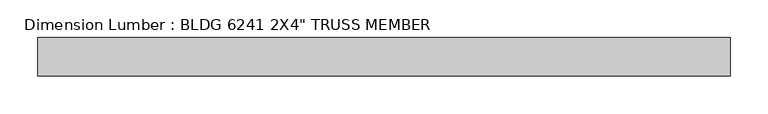
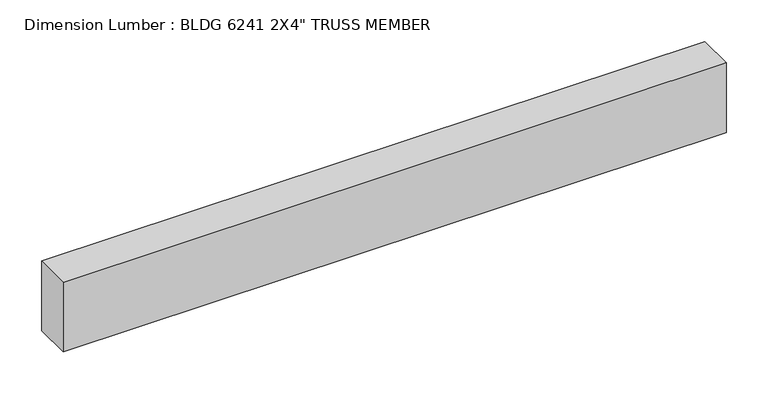
"""IFC4 building model written with IfcOpenShell, lengths in millimetres: beam geometry."""

from ifc_helpers import new_model, si_unit, frame, origin, place, context, project, spatial, polyline, outline, extrude, source, transform, mapped, element, save


def beam_60fbd3f3(model_context):
    return source(origin(), model_context, "Body", "SweptSolid", [
        extrude(outline(polyline([(457.2, 25.4), (457.2, -25.4), (-457.2, -25.4), (-457.2, 25.4), (457.2, 25.4)])), frame((0.0, 0.0, -50.8), z_axis=(0.0, 0.0, 1.0), x_axis=(1.0, 0.0, 0.0)), (0.0, 0.0, 1.0), 101.6),
    ])


if __name__ == "__main__":
    model = new_model("IFC4")
    model_context = context("Model", 3, world=origin())
    ifc_project = project(units=[si_unit("LENGTHUNIT", "METRE", prefix="MILLI")], contexts=[model_context])
    site = spatial("IfcSite", under=ifc_project)
    building = spatial("IfcBuilding", under=site)
    placement = place(None, origin())
    beam_shape = beam_60fbd3f3(model_context)
    element("IfcBeam", 1, ObjectType="Dimension Lumber : BLDG 6241 2X4\" TRUSS MEMBER", at=placement, inside=building, context=model_context, shape_type="MappedRepresentation", body=[
        mapped(beam_shape, transform((0.0, 0.0, 0.0), x_axis=(1.0, 0.0, 0.0), y_axis=(0.0, 1.0, 0.0), z_axis=(0.0, 0.0, 1.0))),
    ])
    save(model, "model.ifc")

# Revit data of these elements
# Type "Dimension Lumber : BLDG 6241 2X4\" TRUSS MEMBER"
#   Assembly Code = "B10"
#   A = 0.273472 SF
#   Length [instance default] = 5' - 0"
#   b = 0' - 2"
#   d = 0' - 4"
#   Structural Material [instance default] = Softwood, Lumber
# Element 1 (IfcBeam, "Dimension Lumber : BLDG 6241 2X4\" TRUSS MEMBER")
#   Materials on its faces: "Softwood, Lumber"
# Materials
#   "Softwood, Lumber": class "Wood", colour RGB 223 192 134, transparency 0, Description = "Pinus Echinata", Cost = 0
